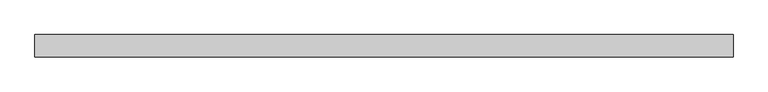
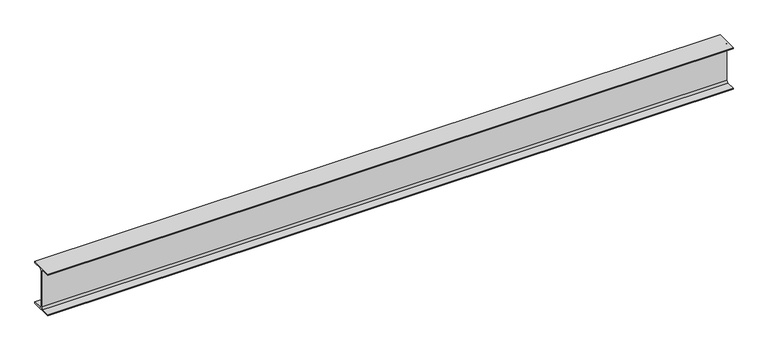
"""IFC4 building model written with IfcOpenShell, lengths in millimetres: beam geometry, 0912_Steel Framing_H-KSD3502 : H_SB_ASB_H-400x200x8x13."""

from ifc_helpers import new_model, si_unit, point, frame, frame_2d, origin, place, context, project, spatial, polyline, circle_curve, trimmed, segment, composite_curve, outline, extrude, source, transform, mapped, element, save


def beam_f29263d3(model_context):
    return source(origin(), model_context, "Body", "SweptSolid", [
        extrude(outline(composite_curve([segment(polyline([(100.0, -187.0), (100.0, -200.0), (-100.0, -200.0), (-100.0, -187.0), (-20.0, -187.0)]), True, "CONTINUOUS"), segment(trimmed(circle_curve(frame_2d((-20.0, -171.0)), 16.0), [point((-20.0, -187.0))], [point((-4.0, -171.0))], True, "CARTESIAN"), True, "CONTINUOUS"), segment(polyline([(-4.0, -171.0), (-4.0, 171.0)]), True, "CONTINUOUS"), segment(trimmed(circle_curve(frame_2d((-20.0, 171.0)), 16.0), [point((-4.0, 171.0))], [point((-20.0, 187.0))], True, "CARTESIAN"), True, "CONTINUOUS"), segment(polyline([(-20.0, 187.0), (-100.0, 187.0), (-100.0, 200.0), (100.0, 200.0), (100.0, 187.0), (20.0, 187.0)]), True, "CONTINUOUS"), segment(trimmed(circle_curve(frame_2d((20.0, 171.0)), 16.0), [point((20.0, 187.0))], [point((4.0, 171.0))], True, "CARTESIAN"), True, "CONTINUOUS"), segment(polyline([(4.0, 171.0), (4.0, -171.0)]), True, "CONTINUOUS"), segment(trimmed(circle_curve(frame_2d((20.0, -171.0)), 16.0), [point((4.0, -171.0))], [point((20.0, -187.0))], True, "CARTESIAN"), True, "CONTINUOUS"), segment(polyline([(20.0, -187.0), (100.0, -187.0)]), True, "CONTINUOUS")], self_intersect=False)), frame((-3154.8, 0.0, 0.0), z_axis=(1.0, 0.0, 0.0), x_axis=(0.0, 1.0, 0.0)), (0.0, 0.0, 1.0), 6192.1),
    ])


if __name__ == "__main__":
    model = new_model("IFC4")
    model_context = context("Model", 3, world=origin())
    ifc_project = project(units=[si_unit("LENGTHUNIT", "METRE", prefix="MILLI")], contexts=[model_context])
    site = spatial("IfcSite", under=ifc_project)
    building = spatial("IfcBuilding", under=site)
    placement = place(None, origin())
    beam_shape = beam_f29263d3(model_context)
    element("IfcBeam", 1, ObjectType="0912_Steel Framing_H-KSD3502 : H_SB_ASB_H-400x200x8x13", at=placement, inside=building, context=model_context, shape_type="MappedRepresentation", body=[
        mapped(beam_shape, transform((0.0, 0.0, 0.0), x_axis=(1.0, 0.0, 0.0), y_axis=(0.0, 1.0, 0.0), z_axis=(0.0, 0.0, 1.0))),
    ])
    save(model, "model.ifc")

# Revit data of these elements
# Type "0912_Steel Framing_H-KSD3502 : H_SB_ASB_H-400x200x8x13"
#   H_WM Code_1 = "S01AA002-00001 | Main Steel Structure Fabrication Work | Shelter/Building | Medium Steel - Standard (90KG/M>Weight≥30KG/M) | Material: (   )"
#   H_WM Code_2 = "S03AA028-00001 | Main Steel Structure Erection Work | Shelter/Building | Medium Steel (90KG/M>Weight≥30KG/M) | Material: (   )"
#   H_WM Code_3 = "S01AA010-00001 | Main Steel Structure Fabrication Work | Shelter/Building | Steel Painting/Coating | for Non-Fireproofed Steel Surface, Surface Preparation, Primer, Second & Final Coat | Material: (   )"
#   H_Q'ty Cal Type Tag = "SB-Q2"
#   Width = 20.0 cm
#   Web Thickness = 0.8 cm
#   Web Fillet = 1.6 cm
#   Warping Constant = 649000.0 cm⁶
#   W = 0
#   Torsional Moment of Inertia = 35.8981 cm⁴
#   Section Area = 84.12 cm²
#   Plastic Modulus weak axis = 268.0 cm³
#   Plastic Modulus strong axis = 1330.0 cm³
#   Perimeter = 1.56 m²/m
#   Nominal Weight = 66.00 kgf/m
#   Moment of Inertia weak axis = 1740.00 cm⁴
#   Moment of Inertia strong axis = 23700.00 cm⁴
#   Height = 40.0 cm
#   Flange Thickness = 1.3 cm
#   Elastic Modulus weak axis = 174.0 cm³
#   Elastic Modulus strong axis = 1190.0 cm³
#   Centroid Vertical = 20.0 cm
#   Centroid Horizontal = 10.0 cm
#   Ix = 237000000
#   Length [instance default] = 1.5240 m
#   Zx = 1330000
#   b = 0.2000 m
#   h = 0.4000 m
#   r = 0.0160 m
#   s = 0.0080 m
#   t = 0.0130 m
#   A = 0.008412 m²
#   Structural Material [instance default] = Steel, 45-345
#   Assembly Code = ""
# Element 1 (IfcBeam, "0912_Steel Framing_H-KSD3502 : H_SB_ASB_H-400x200x8x13")
#   Structural Material = none
# Materials
#   "Steel, 45-345": class "Metal", colour RGB 189 187 185, transparency 0, Description = "Steel 345 MPa", Cost = 0
